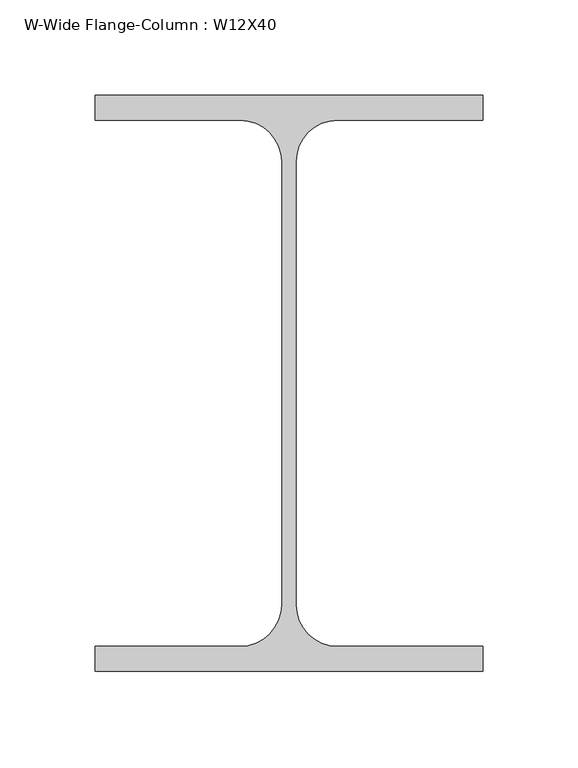
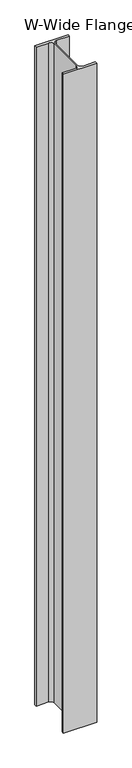
"""IFC4 building model written with IfcOpenShell, lengths in millimetres: column geometry, W-Wide Flange-Column : W12X40."""

from ifc_helpers import new_model, si_unit, point, frame, frame_2d, origin, place, context, project, spatial, polyline, circle_curve, trimmed, segment, composite_curve, outline, extrude, source, transform, mapped, element, save


def w_wide_flange_column_w12x40_e039960b(model_context):
    return source(origin(), model_context, "Body", "SweptSolid", [
        extrude(outline(composite_curve([segment(polyline([(101.727, 151.13), (101.727, 138.049), (25.5905, 138.049)]), True, "CONTINUOUS"), segment(trimmed(circle_curve(frame_2d((25.5905, 116.205)), 21.844), [point((25.5905, 138.049))], [point((3.7465, 116.205))], True, "CARTESIAN"), True, "CONTINUOUS"), segment(polyline([(3.7465, 116.205), (3.7465, -116.205)]), True, "CONTINUOUS"), segment(trimmed(circle_curve(frame_2d((25.5905, -116.205)), 21.844), [point((3.7465, -116.205))], [point((25.5905, -138.049))], True, "CARTESIAN"), True, "CONTINUOUS"), segment(polyline([(25.5905, -138.049), (101.727, -138.049), (101.727, -151.13), (-101.727, -151.13), (-101.727, -138.049), (-25.5905, -138.049)]), True, "CONTINUOUS"), segment(trimmed(circle_curve(frame_2d((-25.5905, -116.205)), 21.844), [point((-25.5905, -138.049))], [point((-3.7465, -116.205))], True, "CARTESIAN"), True, "CONTINUOUS"), segment(polyline([(-3.7465, -116.205), (-3.7465, 116.205)]), True, "CONTINUOUS"), segment(trimmed(circle_curve(frame_2d((-25.5905, 116.205)), 21.844), [point((-3.7465, 116.205))], [point((-25.5905, 138.049))], True, "CARTESIAN"), True, "CONTINUOUS"), segment(polyline([(-25.5905, 138.049), (-101.727, 138.049), (-101.727, 151.13), (101.727, 151.13)]), True, "CONTINUOUS")], self_intersect=False)), frame((0.0, 0.0, 23317.2), z_axis=(0.0, 0.0, 1.0), x_axis=(1.0, 0.0, 0.0)), (0.0, 0.0, 1.0), 4267.2),
    ])


if __name__ == "__main__":
    model = new_model("IFC4")
    model_context = context("Model", 3, world=origin())
    ifc_project = project(units=[si_unit("LENGTHUNIT", "METRE", prefix="MILLI")], contexts=[model_context])
    site = spatial("IfcSite", under=ifc_project)
    building = spatial("IfcBuilding", under=site)
    placement = place(None, origin())
    w_wide_flange_column_w12x40_shape = w_wide_flange_column_w12x40_e039960b(model_context)
    element("IfcColumn", 1, ObjectType="W-Wide Flange-Column : W12X40", at=placement, inside=building, context=model_context, shape_type="MappedRepresentation", body=[
        mapped(w_wide_flange_column_w12x40_shape, transform((0.0, 0.0, 0.0), x_axis=(1.0, 0.0, 0.0), y_axis=(0.0, 1.0, 0.0), z_axis=(0.0, 0.0, 1.0))),
    ])
    save(model, "model.ifc")

# Revit data of these elements
# Type "W-Wide Flange-Column : W12X40"
#   Assembly Code = "B10"
#   W = 40
#   bf = 0' - 8.01"
#   d = 0' - 11.9"
#   k = 0' - 1 3/8"
#   kr = 0' - 0.86"
#   tf = 0' - 0.515"
#   tw = 0' - 0.295"
#   A = 0.08125 SF
#   Structural Material [instance default] = Steel ASTM A992
# Element 1 (IfcColumn, "W-Wide Flange-Column : W12X40")
#   Materials on its faces: "Steel ASTM A992"
# Materials
#   "Steel ASTM A992": class "Metal", colour RGB 199 199 199, transparency 0, Description = "Structural steel 50ksi", Cost = 0
